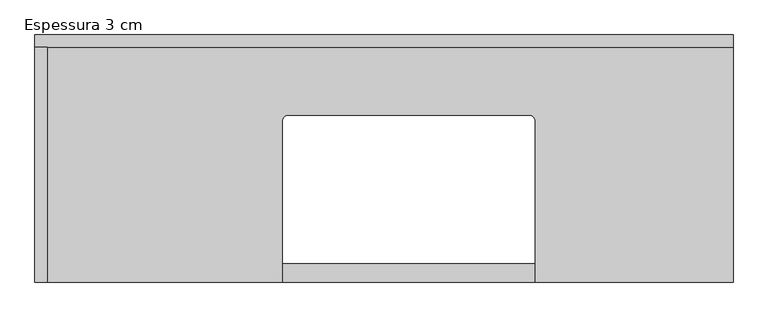
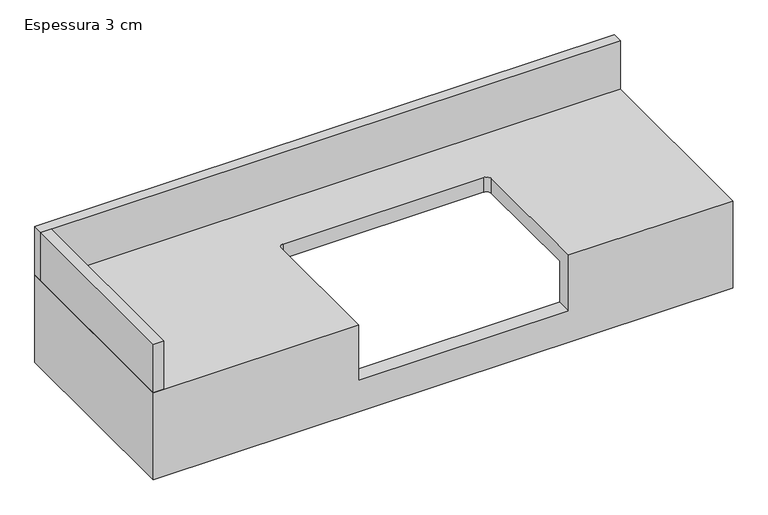
"""IFC4 building model written with IfcOpenShell, lengths in millimetres: furniture geometry, CC_BANCADA BANHEIRO COM CUBA_CANTO RETO : Espessura 3 cm."""

from ifc_helpers import new_model, si_unit, frame, origin, place, context, project, spatial, polyline, circle_curve, outline, extrude, source, transform, mapped, element, save
from ifc_brep_helpers import plane_surface, revolved_surface, advanced_brep


def espessura_3_cm_50a133d0(model_context):
    return source(origin(), model_context, "Body", "SolidModel", [
        advanced_brep(
        [(750.0, 300.0, 860.0), (-380.0, 300.0, 860.0), (-380.0, -100.0, 860.0), (20.0, -100.0, 860.0), (20.0, 160.0, 860.0), (30.0, 170.0, 860.0), (420.0, 170.0, 860.0), (430.0, 160.0, 860.0), (430.0, -100.0, 860.0), (750.0, -100.0, 860.0), (750.0, 300.0, 680.0), (720.0, 300.0, 680.0), (720.0, 300.0, 830.0), (-350.0, 300.0, 830.0), (-350.0, 300.0, 680.0), (-380.0, 300.0, 680.0), (-380.0, -100.0, 680.0), (750.0, -100.0, 680.0), (430.0, -100.0, 745.0), (20.0, -100.0, 745.0), (720.0, -70.0, 830.0), (430.0, -70.0, 830.0), (430.0, 160.0, 830.0), (420.0, 170.0, 830.0), (30.0, 170.0, 830.0), (20.0, 160.0, 830.0), (20.0, -70.0, 830.0), (-350.0, -70.0, 830.0), (-350.0, -70.0, 680.0), (20.0, -70.0, 745.0), (430.0, -70.0, 745.0), (720.0, -70.0, 680.0)],
        [
            (0, 1),
            (1, 2),
            (2, 3),
            (3, 4),
            (4, 5, circle_curve(frame((30.0, 160.0, 860.0), z_axis=(0.0, 0.0, -1.0), x_axis=(0.0, 1.0, 0.0)), 10.0)),
            (5, 6),
            (6, 7, circle_curve(frame((420.0, 160.0, 860.0), z_axis=(0.0, 0.0, -1.0), x_axis=(0.0, 1.0, 0.0)), 10.0)),
            (7, 8),
            (8, 9),
            (9, 0),
            (0, 10),
            (10, 11),
            (11, 12),
            (12, 13),
            (13, 14),
            (14, 15),
            (15, 1),
            (15, 16),
            (16, 2),
            (16, 17),
            (17, 9),
            (8, 18),
            (18, 19),
            (19, 3),
            (17, 10),
            (12, 20),
            (20, 21),
            (21, 22),
            (22, 23, circle_curve(frame((420.0, 160.0, 830.0), z_axis=(0.0, 0.0, 1.0), x_axis=(0.0, 1.0, 0.0)), 10.0)),
            (23, 24),
            (24, 25, circle_curve(frame((30.0, 160.0, 830.0), z_axis=(0.0, 0.0, 1.0), x_axis=(0.0, 1.0, 0.0)), 10.0)),
            (25, 26),
            (26, 27),
            (27, 13),
            (27, 28),
            (28, 14),
            (26, 29),
            (29, 30),
            (30, 21),
            (20, 31),
            (31, 28),
            (11, 31),
            (5, 24),
            (23, 6),
            (18, 30),
            (29, 19),
            (4, 25),
            (7, 22),
        ],
        [
            plane_surface(frame((-380.0, 300.0, 860.0), z_axis=(0.0, 0.0, 1.0), x_axis=(-1.0, 0.0, 0.0))),
            plane_surface(frame((750.0, 300.0, 860.0), z_axis=(0.0, 1.0, 0.0), x_axis=(0.0, 0.0, -1.0))),
            plane_surface(frame((-380.0, 300.0, 860.0), z_axis=(-1.0, 0.0, 0.0), x_axis=(0.0, 0.0, -1.0))),
            plane_surface(frame((-380.0, -100.0, 860.0), z_axis=(0.0, -1.0, 0.0), x_axis=(0.0, 0.0, -1.0))),
            plane_surface(frame((750.0, -100.0, 860.0), z_axis=(1.0, 0.0, 0.0), x_axis=(0.0, 0.0, -1.0))),
            plane_surface(frame((-350.0, 300.0, 830.0), z_axis=(0.0, 0.0, -1.0), x_axis=(-1.0, 0.0, 0.0))),
            plane_surface(frame((-350.0, 300.0, 830.0), z_axis=(1.0, 0.0, 0.0), x_axis=(0.0, 0.0, -1.0))),
            plane_surface(frame((-350.0, -70.0, 830.0), z_axis=(0.0, 1.0, 0.0), x_axis=(0.0, 0.0, -1.0))),
            plane_surface(frame((720.0, -70.0, 830.0), z_axis=(-1.0, 0.0, 0.0), x_axis=(0.0, 0.0, -1.0))),
            plane_surface(frame((750.0, -100.0, 680.0), z_axis=(0.0, 0.0, -1.0), x_axis=(0.0, 1.0, 0.0))),
            plane_surface(frame((30.0, 170.0, 745.0), z_axis=(0.0, -1.0, 0.0), x_axis=(0.0, 0.0, 1.0))),
            plane_surface(frame((420.0, 170.0, 745.0), z_axis=(0.0, 0.0, 1.0), x_axis=(1.0, 0.0, 0.0))),
            revolved_surface(polyline([(30.0, 170.0, 830.0), (30.0, 170.0, 860.0)]), (30.0, 160.0, 900.0), (0.0, 0.0, -1.0)),
            plane_surface(frame((20.0, -230.0, 745.0), z_axis=(1.0, 0.0, 0.0), x_axis=(0.0, 0.0, 1.0))),
            plane_surface(frame((430.0, 160.0, 745.0), z_axis=(-1.0, 0.0, 0.0), x_axis=(0.0, 0.0, 1.0))),
            revolved_surface(polyline([(420.0, 170.0, 830.0), (420.0, 170.0, 860.0)]), (420.0, 160.0, 900.0), (0.0, 0.0, -1.0)),
        ],
        [
            (0, [[1, 2, 3, 4, 5, 6, 7, 8, 9, 10]]),
            (1, [[-1, 11, 12, 13, 14, 15, 16, 17]]),
            (2, [[-2, -17, 18, 19]]),
            (3, [[-3, -19, 20, 21, -9, 22, 23, 24]]),
            (4, [[-10, -21, 25, -11]]),
            (5, [[26, 27, 28, 29, 30, 31, 32, 33, 34, -14]]),
            (6, [[-34, 35, 36, -15]]),
            (7, [[-33, 37, 38, 39, -27, 40, 41, -35]]),
            (8, [[-26, -13, 42, -40]]),
            (9, [[-12, -25, -20, -18, -16, -36, -41, -42]]),
            (10, [[-6, 43, -30, 44]]),
            (11, [[-23, 45, -38, 46]]),
            (12, [[-5, 47, -31, -43]]),
            (13, [[-4, -24, -46, -37, -32, -47]]),
            (14, [[-8, 48, -28, -39, -45, -22]]),
            (15, [[-7, -44, -29, -48]]),
        ],
    ),
        extrude(outline(polyline([(-360.0, -100.0), (-380.0, -100.0), (-380.0, 280.0), (-360.0, 280.0), (-360.0, -100.0)])), frame((0.0, 0.0, 860.0), z_axis=(0.0, 0.0, 1.0), x_axis=(1.0, 0.0, 0.0)), (0.0, 0.0, 1.0), 100.0),
        extrude(outline(polyline([(750.0, 300.0), (750.0, 280.0), (-380.0, 280.0), (-380.0, 300.0), (750.0, 300.0)])), frame((0.0, 0.0, 860.0), z_axis=(0.0, 0.0, 1.0), x_axis=(1.0, 0.0, 0.0)), (0.0, 0.0, 1.0), 100.0),
    ])


if __name__ == "__main__":
    model = new_model("IFC4")
    model_context = context("Model", 3, world=origin())
    ifc_project = project(units=[si_unit("LENGTHUNIT", "METRE", prefix="MILLI")], contexts=[model_context])
    site = spatial("IfcSite", under=ifc_project)
    building = spatial("IfcBuilding", under=site)
    placement = place(None, origin())
    espessura_3_cm_shape = espessura_3_cm_50a133d0(model_context)
    element("IfcFurniture", 1, ObjectType="CC_BANCADA BANHEIRO COM CUBA_CANTO RETO : Espessura 3 cm", at=placement, inside=building, context=model_context, shape_type="MappedRepresentation", body=[
        mapped(espessura_3_cm_shape, transform((0.0, 0.0, 0.0), x_axis=(1.0, 0.0, 0.0), y_axis=(0.0, 1.0, 0.0), z_axis=(0.0, 0.0, 1.0))),
    ])
    save(model, "model.ifc")

# Revit data of these elements
# Type "CC_BANCADA BANHEIRO COM CUBA_CANTO RETO : Espessura 3 cm"
#   Uso HS [instance default] = ""
#   h TESTEIRA AUX [instance default] = 0.15 m
#   Altura testeira [instance default] = 0.15 m
#   Altura rodapia [instance default] = 0.10 m
#   Espessura rodapia [instance default] = 0.02 m
#   Prof/2 [instance default] = 0.20 m
#   Offset cuba esquerda [instance default] = 0.40 m
#   Depth [instance default] = 1.20 m
#   Width [instance default] = 0.40 m
#   Espessura bancada = 0.03 m
#   Comprimento [instance default] = 1.20 m
#   Height [instance default] = 0.86 m
#   Testeira [instance default] = yes
#   Rodapia fundo [instance default] = no
#   Rodapia esquerda [instance default] = no
#   Rodapia direita [instance default] = no
#   Material porta-toalha [instance default] = .CROMADO
#   Material hidráulico [instance default] = .CROMADO
#   Material cuba [instance default] = .PORCELANA BRANCA
#   Material bancada [instance default] = .GRANITO_BRANCO_ITAUNAS
#   Assembly Code = ""
# Element 1 (IfcFurniture, "CC_BANCADA BANHEIRO COM CUBA_CANTO RETO : Espessura 3 cm")
#   Uso HS = "BANHO SUÍTE 2"
#   Depth = 1.13 m
#   Comprimento = 1.13 m
#   Rodapia fundo = yes
#   Rodapia esquerda = yes
#   Materials on its faces: ".GRANITO_BRANCO_ITAUNAS"
# Materials
#   ".CROMADO": class "CC_METAIS", colour RGB 211 223 226, transparency 0, Cost = 0
#   ".PORCELANA BRANCA": class "CC_PORCELANA", colour RGB 230 230 230, transparency 0, Cost = 0
#   ".GRANITO_BRANCO_ITAUNAS": class ".CC_PEDRA REVEST.", colour RGB 202 195 174, transparency 0, Description = "Revestimento em granito", Cost = 0
